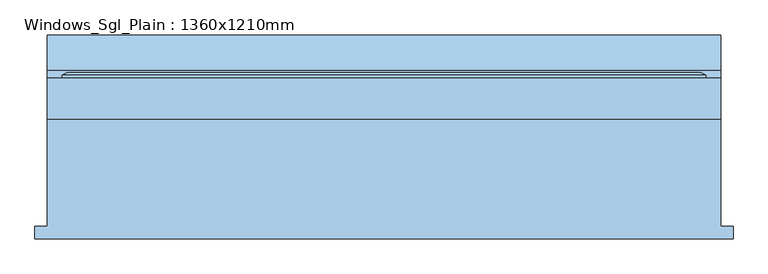
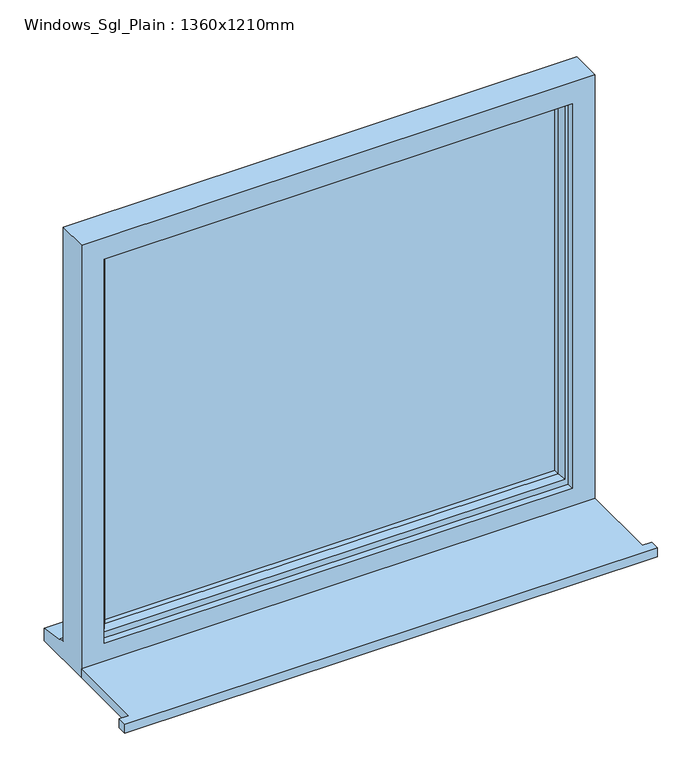
"""IFC4 building model written with IfcOpenShell, lengths in millimetres: window geometry, Windows_Sgl_Plain : 1360x1210mm."""

from ifc_helpers import new_model, si_unit, frame, origin, place, context, project, spatial, polyline, outline, extrude, faceted_brep, source, transform, mapped, element, save


def windows_sgl_plain_1360x1210mm_bb3badfb(model_context):
    return source(origin(), model_context, "Body", "SolidModel", [
        extrude(outline(polyline([(-705.0, -191.5434322), (-705.0, -166.5434322), (-680.0, -166.5434322), (-680.0, 50.4565678), (680.0, 50.4565678), (680.0, -166.5434322), (705.0, -166.5434322), (705.0, -191.5434322), (-705.0, -191.5434322)])), frame((0.0, 0.0, 900.0), z_axis=(0.0, 0.0, 1.0), x_axis=(1.0, 0.0, 0.0)), (0.0, 0.0, 1.0), 25.0),
        faceted_brep([(-680.0, 50.4565678, 900.0), (680.0, 50.4565678, 900.0), (680.0, 50.4565678, 2110.0), (-680.0, 50.4565678, 2110.0), (-620.0, 50.4565678, 2050.0), (620.0, 50.4565678, 2050.0), (620.0, 50.4565678, 975.0), (-620.0, 50.4565678, 975.0), (-680.0, 133.4565678, 2110.0), (-680.0, 133.4565678, 951.0), (-680.0, 148.4565678, 949.68767), (-680.0, 148.4565678, 944.7449676), (-680.0, 220.9565678, 933.8088847), (-680.0, 220.9565678, 900.0), (680.0, 133.4565678, 2110.0), (680.0, 133.4565678, 951.0), (-640.0, 133.4565678, 2070.0), (-640.0, 133.4565678, 963.0), (640.0, 133.4565678, 963.0), (640.0, 133.4565678, 2070.0), (-640.0, 68.4565678, 2070.0), (-640.0, 68.4565678, 963.0), (640.0, 68.4565678, 2070.0), (640.0, 68.4565678, 963.0), (-620.0, 68.4565678, 2050.0), (-620.0, 68.4565678, 975.0), (620.0, 68.4565678, 975.0), (620.0, 68.4565678, 2050.0), (680.0, 220.9565678, 900.0), (680.0, 220.9565678, 933.8088847), (680.0, 148.4565678, 944.7449676), (680.0, 148.4565678, 949.68767)], [[[0, 1, 2, 3], [4, 5, 6, 7]], [[0, 3, 8, 9, 10, 11, 12, 13]], [[9, 8, 14, 15], [16, 17, 18, 19]], [[17, 16, 20, 21]], [[20, 22, 23, 21], [24, 25, 26, 27]], [[24, 4, 7, 25]], [[3, 2, 14, 8]], [[16, 19, 22, 20]], [[5, 4, 24, 27]], [[15, 14, 2, 1, 28, 29, 30, 31]], [[19, 18, 23, 22]], [[5, 27, 26, 6]], [[28, 1, 0, 13]], [[29, 28, 13, 12]], [[30, 29, 12, 11]], [[31, 30, 11, 10]], [[15, 31, 10, 9]], [[21, 23, 18, 17]], [[7, 6, 26, 25]]]),
        extrude(outline(polyline([(610.0, 97.4565678), (-610.0, 97.4565678), (-610.0, 121.4565678), (610.0, 121.4565678), (610.0, 97.4565678)])), frame((0.0, 0.0, 993.0), z_axis=(0.0, 0.0, 1.0), x_axis=(1.0, 0.0, 0.0)), (0.0, 0.0, 1.0), 1047.0),
        faceted_brep([(-650.0, 133.4565678, 2080.0), (-650.0, 139.2300705, 2080.0), (-650.0, 139.2300705, 953.0), (-650.0, 133.4565678, 953.0), (-640.0, 68.4565678, 2070.0), (-640.0, 133.4565678, 2070.0), (-640.0, 133.4565678, 963.0), (-640.0, 68.4565678, 963.0), (-600.0, 82.9494677, 2030.0), (-610.1480377, 68.4565678, 2040.1480377), (-610.1480377, 68.4565678, 992.8519623), (-600.0, 82.9494677, 1003.0), (-600.0, 97.4565678, 2030.0), (-600.0, 97.4565678, 1003.0), (-610.0, 121.4565678, 2040.0), (-610.0, 97.4565678, 2040.0), (-610.0, 97.4565678, 993.0), (-610.0, 121.4565678, 993.0), (-600.0, 139.2300705, 2030.0), (-600.0, 121.4565678, 2030.0), (-600.0, 121.4565678, 1003.0), (-600.0, 139.2300705, 1003.0), (-617.4457548, 145.0035732, 2047.4457548), (-617.4457548, 145.0035732, 985.5542452), (-639.2153903, 145.0035732, 2069.2153903), (-639.2153903, 145.0035732, 963.7846097), (650.0, 139.2300705, 953.0), (650.0, 133.4565678, 953.0), (640.0, 133.4565678, 963.0), (640.0, 68.4565678, 963.0), (610.1480377, 68.4565678, 992.8519623), (600.0, 82.9494677, 1003.0), (600.0, 97.4565678, 1003.0), (610.0, 97.4565678, 993.0), (610.0, 121.4565678, 993.0), (600.0, 121.4565678, 1003.0), (600.0, 139.2300705, 1003.0), (617.4457548, 145.0035732, 985.5542452), (639.2153903, 145.0035732, 963.7846097), (650.0, 139.2300705, 2080.0), (650.0, 133.4565678, 2080.0), (640.0, 133.4565678, 2070.0), (640.0, 68.4565678, 2070.0), (610.1480377, 68.4565678, 2040.1480377), (600.0, 82.9494677, 2030.0), (600.0, 97.4565678, 2030.0), (610.0, 97.4565678, 2040.0), (610.0, 121.4565678, 2040.0), (600.0, 121.4565678, 2030.0), (600.0, 139.2300705, 2030.0), (617.4457548, 145.0035732, 2047.4457548), (639.2153903, 145.0035732, 2069.2153903)], [[[0, 1, 2, 3]], [[4, 5, 6, 7]], [[8, 9, 10, 11]], [[12, 8, 11, 13]], [[14, 15, 16, 17]], [[18, 19, 20, 21]], [[22, 18, 21, 23]], [[1, 24, 25, 2]], [[3, 2, 26, 27]], [[7, 6, 28, 29]], [[11, 10, 30, 31]], [[13, 11, 31, 32]], [[17, 16, 33, 34]], [[21, 20, 35, 36]], [[23, 21, 36, 37]], [[2, 25, 38, 26]], [[27, 26, 39, 40]], [[29, 28, 41, 42]], [[31, 30, 43, 44]], [[32, 31, 44, 45]], [[34, 33, 46, 47]], [[36, 35, 48, 49]], [[37, 36, 49, 50]], [[26, 38, 51, 39]], [[40, 39, 1, 0]], [[3, 27, 40, 0], [5, 41, 28, 6]], [[42, 41, 5, 4]], [[7, 29, 42, 4], [9, 43, 30, 10]], [[44, 43, 9, 8]], [[45, 44, 8, 12]], [[15, 46, 33, 16], [13, 32, 45, 12]], [[47, 46, 15, 14]], [[17, 34, 47, 14], [19, 48, 35, 20]], [[49, 48, 19, 18]], [[50, 49, 18, 22]], [[24, 51, 38, 25], [23, 37, 50, 22]], [[39, 51, 24, 1]]]),
    ])


if __name__ == "__main__":
    model = new_model("IFC4")
    model_context = context("Model", 3, world=origin())
    ifc_project = project(units=[si_unit("LENGTHUNIT", "METRE", prefix="MILLI")], contexts=[model_context])
    site = spatial("IfcSite", under=ifc_project)
    building = spatial("IfcBuilding", under=site)
    placement = place(None, origin())
    windows_sgl_plain_1360x1210mm_shape = windows_sgl_plain_1360x1210mm_bb3badfb(model_context)
    element("IfcWindow", 1, ObjectType="Windows_Sgl_Plain : 1360x1210mm", at=placement, inside=building, context=model_context, shape_type="MappedRepresentation", body=[
        mapped(windows_sgl_plain_1360x1210mm_shape, transform((0.0, 0.0, 0.0), x_axis=(1.0, 0.0, 0.0), y_axis=(0.0, 1.0, 0.0), z_axis=(0.0, 0.0, 1.0))),
    ])
    save(model, "model.ifc")

# Revit data of these elements
# Type "Windows_Sgl_Plain : 1360x1210mm"
#   Type Mark = "47"
#   Operation = "SinglePanel"
#   Construction Type Id = "SGL"
#   Manufacturer = "Revit"
#   Keynote = "L10"
#   Analytic Construction = "Large single-glazed windows"
#   Wrap Layers (Ext) from Ext = 102.5 mm
#   Wrap Layers (Int) from Ext = 177.5 mm
#   Window Board Projection = 25 mm
#   Window Board Extension = 25 mm
#   Visual Light Transmittance = 0.9
#   Solar Heat Gain Coefficient = 0.86
#   Rough Width = 1360 mm
#   Rough Height = 1210 mm
#   Height = 1210 mm
#   Width = 1360 mm
#   Heat Transfer Coefficient (U) = 5.5617 W/(m²·K)
#   Glazing Thickness = 24 mm
#   FrameOffset - External = 50 mm
#   Frame Depth = 65 mm
#   Default Head Height = 2110 mm
#   Cill Depth = 87.5 mm
#   Cavity Closer Width = 50 mm
#   Cavity Closer Offset from Ext = 102.5 mm
#   Cavity Closer Depth = 85 mm
#   Vis - Cavity Closers = yes
#   Define Thermal Properties by = 1
#   Material Trim = Window Frame
#   Material Glass = Glass
#   Material Frame = Window Frame
#   Wall Closure = (empty or 0)
# Element 1 (IfcWindow, "Windows_Sgl_Plain : 1360x1210mm")
#   Materials on its faces: "Window Frame", "Glass"
# Materials
#   "Window Frame": class "Miscellaneous", colour RGB 249 249 249, transparency 0, Keynote = "L10", Cost = 0
#   "Glass": class "Glass", colour RGB 0 128 192, transparency 0.9, Description = "Soda Lime Glass", Cost = 0
